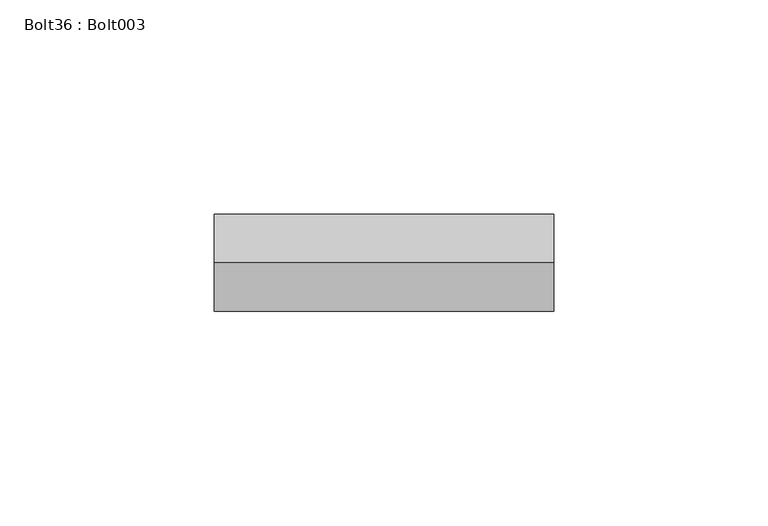
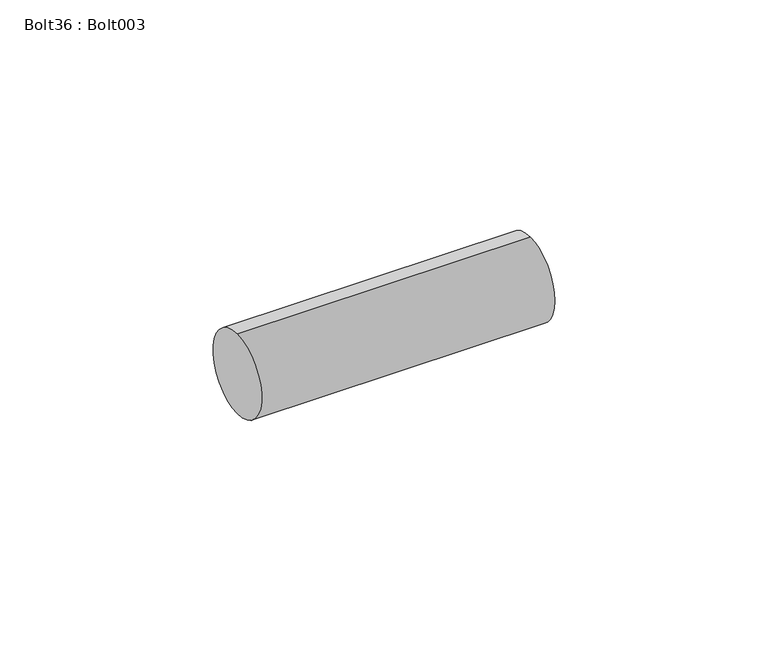
"""IFC4 building model written with IfcOpenShell, lengths in millimetres: proxy geometry, Bolt36 : Bolt003."""

from ifc_helpers import new_model, si_unit, point, frame, frame_2d, origin, place, context, project, spatial, circle_curve, trimmed, segment, composite_curve, outline, extrude, source, transform, mapped, element, save


def bolt36_bolt003_fc88f5ab(model_context):
    return source(origin(), model_context, "Body", "SweptSolid", [
        extrude(outline(composite_curve([segment(trimmed(circle_curve(frame_2d((1896.5882072, 39960.0063132)), 11.4045168), [point((1896.5882072, 39971.41083))], [point((1896.5882072, 39948.6017964))], False, "CARTESIAN"), True, "CONTINUOUS"), segment(trimmed(circle_curve(frame_2d((1896.5882072, 39960.0063132)), 11.4045168), [point((1896.5882072, 39948.6017964))], [point((1896.5882072, 39971.41083))], False, "CARTESIAN"), True, "CONTINUOUS")], self_intersect=False)), frame((10265.0890809, 0.0, 0.0), z_axis=(1.0, 0.0, 0.0), x_axis=(0.0, 1.0, 0.0)), (0.0, 0.0, 1.0), 79.375),
    ])


if __name__ == "__main__":
    model = new_model("IFC4")
    model_context = context("Model", 3, world=origin())
    ifc_project = project(units=[si_unit("LENGTHUNIT", "METRE", prefix="MILLI")], contexts=[model_context])
    site = spatial("IfcSite", under=ifc_project)
    building = spatial("IfcBuilding", under=site)
    placement = place(None, origin())
    bolt36_bolt003_shape = bolt36_bolt003_fc88f5ab(model_context)
    element("IfcBuildingElementProxy", 1, Name="Bolt36 : Bolt003", ObjectType="Bolt36 : Bolt003", at=placement, inside=building, context=model_context, shape_type="MappedRepresentation", body=[
        mapped(bolt36_bolt003_shape, transform((0.0, 0.0, 0.0), x_axis=(1.0, 0.0, 0.0), y_axis=(0.0, 1.0, 0.0), z_axis=(0.0, 0.0, 1.0))),
    ])
    save(model, "model.ifc")

# Revit data of these elements
# Type "Bolt36 : Bolt003"
#   NameOverride = "Bolt003"
# Element 1 (IfcBuildingElementProxy, "Bolt36 : Bolt003")
#   Materials on its faces: "STEEL ANGLE AND ANCHOR BOLT (SEE STRUCT. DWGS)"
# Materials
#   "STEEL ANGLE AND ANCHOR BOLT (SEE STRUCT. DWGS)": class "Unassigned", colour RGB 128 128 128, transparency 0, Cost = 0
